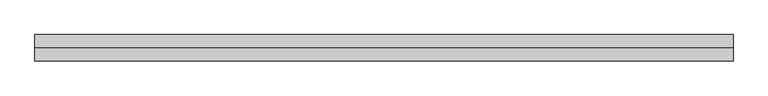
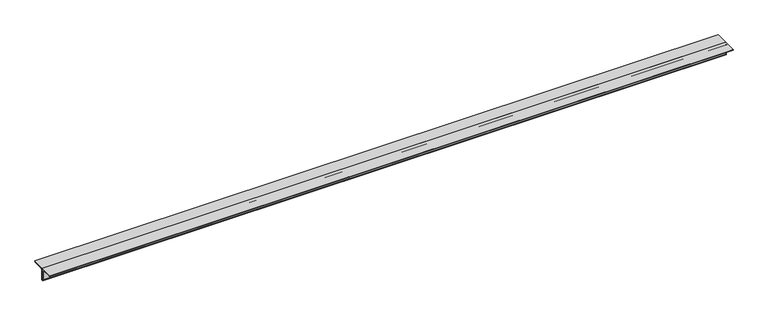
"""IFC4 building model written with IfcOpenShell, lengths in millimetres: member geometry, Steel Framing_2Ls_KS : H_SB_AR_S02_2Ls-100x100x10_VBR1."""

from ifc_helpers import new_model, si_unit, point, frame, frame_2d, origin, place, context, project, spatial, polyline, circle_curve, trimmed, segment, composite_curve, outline, extrude, source, transform, mapped, element, save


def member_42fd508a(model_context):
    return source(origin(), model_context, "Body", "SweptSolid", [
        extrude(outline(composite_curve([segment(polyline([(0.0, 28.2), (0.0, -71.8)]), True, "CONTINUOUS"), segment(trimmed(circle_curve(frame_2d((0.0, -61.8)), 10.0), [point((0.0, -71.8))], [point((-10.0, -61.8))], False, "CARTESIAN"), True, "CONTINUOUS"), segment(polyline([(-10.0, -61.8), (-10.0, 8.2)]), True, "CONTINUOUS"), segment(trimmed(circle_curve(frame_2d((-20.0, 8.2)), 10.0), [point((-10.0, 8.2))], [point((-20.0, 18.2))], True, "CARTESIAN"), True, "CONTINUOUS"), segment(polyline([(-20.0, 18.2), (-90.0, 18.2)]), True, "CONTINUOUS"), segment(trimmed(circle_curve(frame_2d((-90.0, 28.2)), 10.0), [point((-90.0, 18.2))], [point((-100.0, 28.2))], False, "CARTESIAN"), True, "CONTINUOUS"), segment(polyline([(-100.0, 28.2), (0.0, 28.2)]), True, "CONTINUOUS")], self_intersect=False)), frame((-2444.561686, 0.0, 0.0), z_axis=(1.0, 0.0, 0.0), x_axis=(0.0, 1.0, 0.0)), (0.0, 0.0, 1.0), 5283.025664),
        extrude(outline(composite_curve([segment(polyline([(0.0, 28.2), (100.0, 28.2)]), True, "CONTINUOUS"), segment(trimmed(circle_curve(frame_2d((90.0, 28.2)), 10.0), [point((100.0, 28.2))], [point((90.0, 18.2))], False, "CARTESIAN"), True, "CONTINUOUS"), segment(polyline([(90.0, 18.2), (20.0, 18.2)]), True, "CONTINUOUS"), segment(trimmed(circle_curve(frame_2d((20.0, 8.2)), 10.0), [point((20.0, 18.2))], [point((10.0, 8.2))], True, "CARTESIAN"), True, "CONTINUOUS"), segment(polyline([(10.0, 8.2), (10.0, -61.8)]), True, "CONTINUOUS"), segment(trimmed(circle_curve(frame_2d((0.0, -61.8)), 10.0), [point((10.0, -61.8))], [point((0.0, -71.8))], False, "CARTESIAN"), True, "CONTINUOUS"), segment(polyline([(0.0, -71.8), (0.0, 28.2)]), True, "CONTINUOUS")], self_intersect=False)), frame((-2444.561686, 0.0, 0.0), z_axis=(1.0, 0.0, 0.0), x_axis=(0.0, 1.0, 0.0)), (0.0, 0.0, 1.0), 5283.025664),
    ])


if __name__ == "__main__":
    model = new_model("IFC4")
    model_context = context("Model", 3, world=origin())
    ifc_project = project(units=[si_unit("LENGTHUNIT", "METRE", prefix="MILLI")], contexts=[model_context])
    site = spatial("IfcSite", under=ifc_project)
    building = spatial("IfcBuilding", under=site)
    placement = place(None, origin())
    member_shape = member_42fd508a(model_context)
    element("IfcMember", 1, ObjectType="Steel Framing_2Ls_KS : H_SB_AR_S02_2Ls-100x100x10_VBR1", at=placement, inside=building, context=model_context, shape_type="MappedRepresentation", body=[
        mapped(member_shape, transform((0.0, 0.0, 0.0), x_axis=(1.0, 0.0, 0.0), y_axis=(0.0, 1.0, 0.0), z_axis=(0.0, 0.0, 1.0))),
    ])
    save(model, "model.ifc")

# Revit data of these elements
# Type "Steel Framing_2Ls_KS : H_SB_AR_S02_2Ls-100x100x10_VBR1"
#   Type Comments = "MAIN"
#   Type Mark = "VBR1"
#   H_SectionID = "2Ls-100x100x10"
#   Assembly Code = "B10"
#   Legs = "LLBB"
#   H_Ratio for Additional Steel Plate = 0.2
#   W = 0
#   Perimeter = 0.80 m²/m
#   Nominal Weight = 29.80 kgf/m
#   Length [instance default] = 1524 mm
#   Space = 0 mm
#   b = 100 mm
#   d = 100 mm
#   t = 10 mm
#   y = 28.2 mm
#   A = 0.0038 m²
#   Structural Material [instance default] = Steel, 45-345
# Element 1 (IfcMember, "Steel Framing_2Ls_KS : H_SB_AR_S02_2Ls-100x100x10_VBR1")
#   Materials on its faces: "Steel, 45-345"
# Materials
#   "Steel, 45-345": class "Metal", colour RGB 189 187 185, transparency 0, Description = "Steel 345 MPa", Cost = 0
